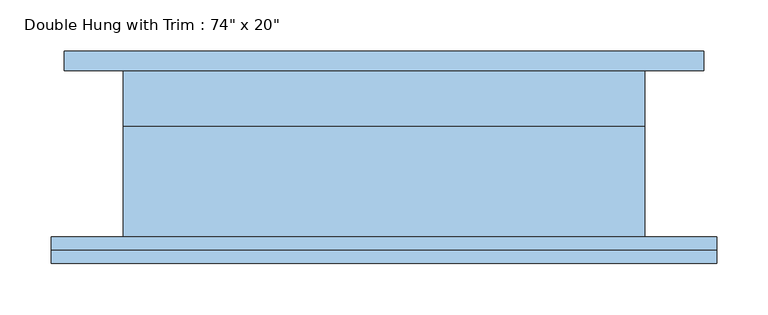
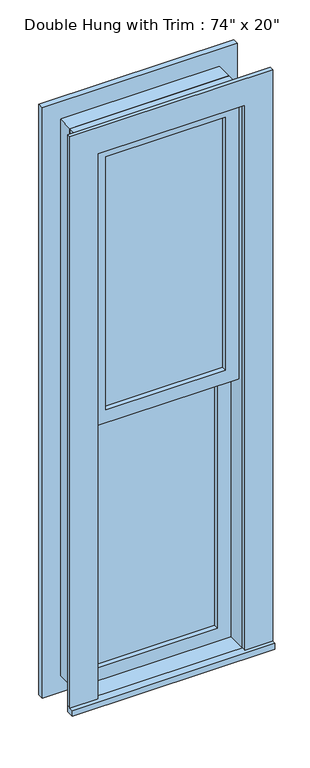
"""IFC4 building model written with IfcOpenShell, lengths in millimetres: window geometry."""

from ifc_helpers import new_model, si_unit, frame, origin, place, context, project, spatial, polyline, outline, extrude, source, transform, mapped, element, save


def window_c3f1e6f6(model_context):
    return source(origin(), model_context, "Body", "SweptSolid", [
        extrude(outline(polyline([(-190.5, -1.5875), (-190.5, 11.1125), (190.5, 11.1125), (190.5, -1.5875), (-190.5, -1.5875)])), frame((0.0, 0.0, 571.5), z_axis=(0.0, 0.0, 1.0), x_axis=(1.0, 0.0, 0.0)), (0.0, 0.0, 1.0), 854.075),
        extrude(outline(polyline([(1470.025, -234.95), (527.05, -234.95), (527.05, 234.95), (1470.025, 234.95), (1470.025, -234.95)]), holes=[polyline([(1425.575, -190.5), (1425.575, 190.5), (571.5, 190.5), (571.5, -190.5), (1425.575, -190.5)])]), frame((0.0, -17.4625, 0.0), z_axis=(0.0, 1.0, 0.0), x_axis=(0.0, 0.0, 1.0)), (0.0, 0.0, 1.0), 44.45),
        extrude(outline(polyline([(-323.85, -106.3625), (-323.85, -80.9625), (323.85, -80.9625), (323.85, -106.3625), (-323.85, -106.3625)])), frame((0.0, 0.0, 508.0), z_axis=(0.0, 0.0, 1.0), x_axis=(1.0, 0.0, 0.0)), (0.0, 0.0, 1.0), 19.05),
        extrude(outline(polyline([(2368.55, -234.95), (2368.55, 234.95), (527.05, 234.95), (527.05, 323.85), (2457.45, 323.85), (2457.45, -323.85), (527.05, -323.85), (527.05, -234.95), (2368.55, -234.95)])), frame((0.0, -93.6625, 0.0), z_axis=(0.0, 1.0, 0.0), x_axis=(0.0, 0.0, 1.0)), (0.0, 0.0, 1.0), 12.7),
        extrude(outline(polyline([(2444.75, 311.15), (2444.75, -311.15), (450.85, -311.15), (450.85, 311.15), (2444.75, 311.15)]), holes=[polyline([(2355.85, 222.25), (539.75, 222.25), (539.75, -222.25), (2355.85, -222.25), (2355.85, 222.25)])]), frame((0.0, 80.9625, 0.0), z_axis=(0.0, 1.0, 0.0), x_axis=(0.0, 0.0, 1.0)), (0.0, 0.0, 1.0), 19.05),
        extrude(outline(polyline([(190.5, -33.3375), (190.5, -46.0375), (-190.5, -46.0375), (-190.5, -33.3375), (190.5, -33.3375)])), frame((0.0, 0.0, 1470.025), z_axis=(0.0, 0.0, 1.0), x_axis=(1.0, 0.0, 0.0)), (0.0, 0.0, 1.0), 854.075),
        extrude(outline(polyline([(2368.55, -234.95), (1425.575, -234.95), (1425.575, 234.95), (2368.55, 234.95), (2368.55, -234.95)]), holes=[polyline([(2324.1, -190.5), (2324.1, 190.5), (1470.025, 190.5), (1470.025, -190.5), (2324.1, -190.5)])]), frame((0.0, -61.9125, 0.0), z_axis=(0.0, 1.0, 0.0), x_axis=(0.0, 0.0, 1.0)), (0.0, 0.0, 1.0), 44.45),
        extrude(outline(polyline([(2387.6, -254.0), (508.0, -254.0), (508.0, 254.0), (2387.6, 254.0), (2387.6, -254.0)]), holes=[polyline([(2355.85, -222.25), (2355.85, 222.25), (539.75, 222.25), (539.75, -222.25), (2355.85, -222.25)])]), frame((0.0, 26.9875, 0.0), z_axis=(0.0, 1.0, 0.0), x_axis=(0.0, 0.0, 1.0)), (0.0, 0.0, 1.0), 53.975),
        extrude(outline(polyline([(2387.6, 254.0), (2387.6, -254.0), (508.0, -254.0), (508.0, 254.0), (2387.6, 254.0)]), holes=[polyline([(2368.55, 234.95), (527.05, 234.95), (527.05, -234.95), (2368.55, -234.95), (2368.55, 234.95)])]), frame((0.0, -80.9625, 0.0), z_axis=(0.0, 1.0, 0.0), x_axis=(0.0, 0.0, 1.0)), (0.0, 0.0, 1.0), 107.95),
    ])


if __name__ == "__main__":
    model = new_model("IFC4")
    model_context = context("Model", 3, world=origin())
    ifc_project = project(units=[si_unit("LENGTHUNIT", "METRE", prefix="MILLI")], contexts=[model_context])
    site = spatial("IfcSite", under=ifc_project)
    building = spatial("IfcBuilding", under=site)
    placement = place(None, origin())
    window_shape = window_c3f1e6f6(model_context)
    element("IfcWindow", 1, ObjectType="Double Hung with Trim : 74\" x 20\"", at=placement, inside=building, context=model_context, shape_type="MappedRepresentation", body=[
        mapped(window_shape, transform((0.0, 0.0, 0.0), x_axis=(1.0, 0.0, 0.0), y_axis=(0.0, 1.0, 0.0), z_axis=(0.0, 0.0, 1.0))),
    ])
    save(model, "model.ifc")

# Revit data of these elements
# Type "Double Hung with Trim : 74\" x 20\""
#   Type Mark = "56"
#   COBie.Type.CreatedBy = "doug.wood@us.ibm.com"
#   COBie.Type.CreatedOn = "2016-04-14T02:07:26"
#   COBie.Type.Name = "Windows_Double Hung with Trim_74\" x 20\"_56"
#   COBie.Type.Category = "23-30 20 17 17 14 : Double-Hung Windows"
#   COBie.Type.Description = "Double Hung with Trim_74\" x 20\""
#   COBie.Type.Manufacturer = ""
#   COBie.Type.ModelNumber = ""
#   Construction Type Id = "GSP4R"
#   Assembly Code = "B2020100"
#   Analytic Construction = "1/8 in Pilkington single glazing"
#   COBie.Type.ReplacementCost = 0
#   Visual Light Transmittance = 0.9
#   Solar Heat Gain Coefficient = 0.78
#   Heat Transfer Coefficient (U) = 3.6886 W/(m²·K)
#   Height = 6' - 2"
#   Default Sill Height = 1' - 8"
#   Trim Projection - Ext. = 0' - 0 1/2"
#   Trim Projection - Int. = 0' - 0 3/4"
#   Trim Width - Exterior = 0' - 3 1/2"
#   Trim Width - Interior = 0' - 3 1/2"
#   Width = 1' - 8"
#   Window Inset = 0' - 0 3/4"
#   COBie.Type = no
#   Glass Pane Material = Glass
#   Sash Material = Sash - White
#   Trim Exterior Material = Trim - White
#   Trim Interior Material = Trim - White
#   Wall Closure = (empty or 0)
# Element 1 (IfcWindow, "Double Hung with Trim : 74\" x 20\"")
#   Materials on its faces: "Sash - White", "Trim - White", "Glass"
# Materials
#   "Glass": class "Glass", colour RGB 0 128 192, transparency 0.75, Description = "Soda Lime Glass", Cost = 0
#   "Sash - White": class "Wood", colour RGB 255 255 255, transparency 0, Cost = 0
#   "Trim - White": class "Wood", colour RGB 255 255 255, transparency 0, Cost = 0
